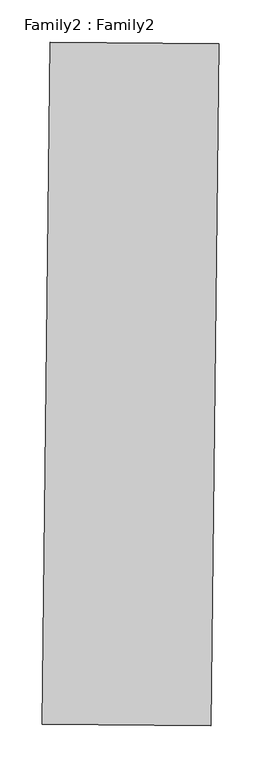
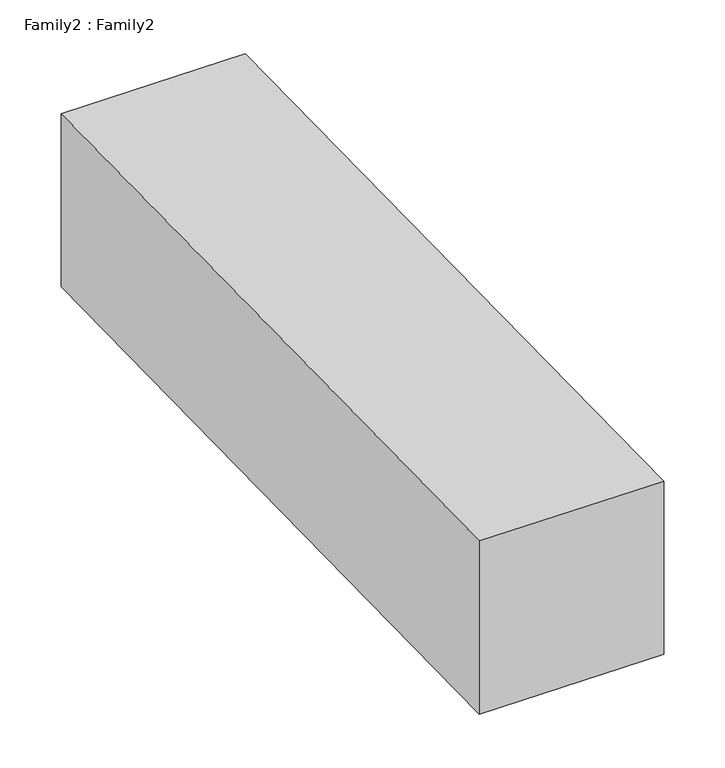
"""IFC4 building model written with IfcOpenShell, lengths in millimetres: proxy geometry, Family2 : Family2."""

from ifc_helpers import new_model, si_unit, origin, place, context, project, spatial, faceted_brep, source, transform, mapped, element, save


def family2_family2_ec7d01cc(model_context):
    return source(origin(), model_context, "Body", "Brep", [
        faceted_brep([(-3948.0215464, -6477.1012252, 1.0945136), (-3948.0215464, -6477.1012252, 201.0945136), (-3938.8212481, -5670.4988974, 202.060409), (-3938.8212481, -5670.4988974, 2.060409), (-3748.0303564, -6478.9784379, 201.0945136), (-3738.8300581, -5672.3761101, 202.060409), (-3748.0303564, -6478.9784379, 1.0945136), (-3738.8300581, -5672.3761101, 2.060409)], [[[0, 1, 2, 3]], [[1, 4, 5, 2]], [[4, 6, 7, 5]], [[6, 0, 3, 7]], [[3, 2, 5, 7]], [[0, 6, 4, 1]]]),
    ])


if __name__ == "__main__":
    model = new_model("IFC4")
    model_context = context("Model", 3, world=origin())
    ifc_project = project(units=[si_unit("LENGTHUNIT", "METRE", prefix="MILLI")], contexts=[model_context])
    site = spatial("IfcSite", under=ifc_project)
    building = spatial("IfcBuilding", under=site)
    placement = place(None, origin())
    family2_family2_shape = family2_family2_ec7d01cc(model_context)
    element("IfcBuildingElementProxy", 1, Name="Family2 : Family2", ObjectType="Family2 : Family2", at=placement, inside=building, context=model_context, shape_type="MappedRepresentation", body=[
        mapped(family2_family2_shape, transform((0.0, 0.0, 0.0), x_axis=(1.0, 0.0, 0.0), y_axis=(0.0, 1.0, 0.0), z_axis=(0.0, 0.0, 1.0))),
    ])
    save(model, "model.ifc")

# Revit data of these elements
# Type "Family2 : Family2"
#   Default Elevation = 0
